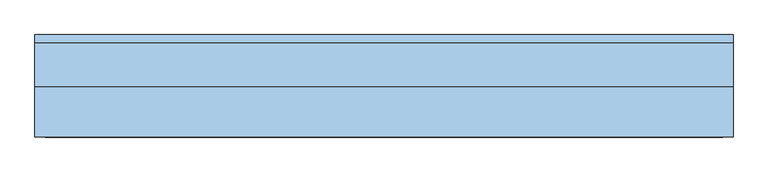
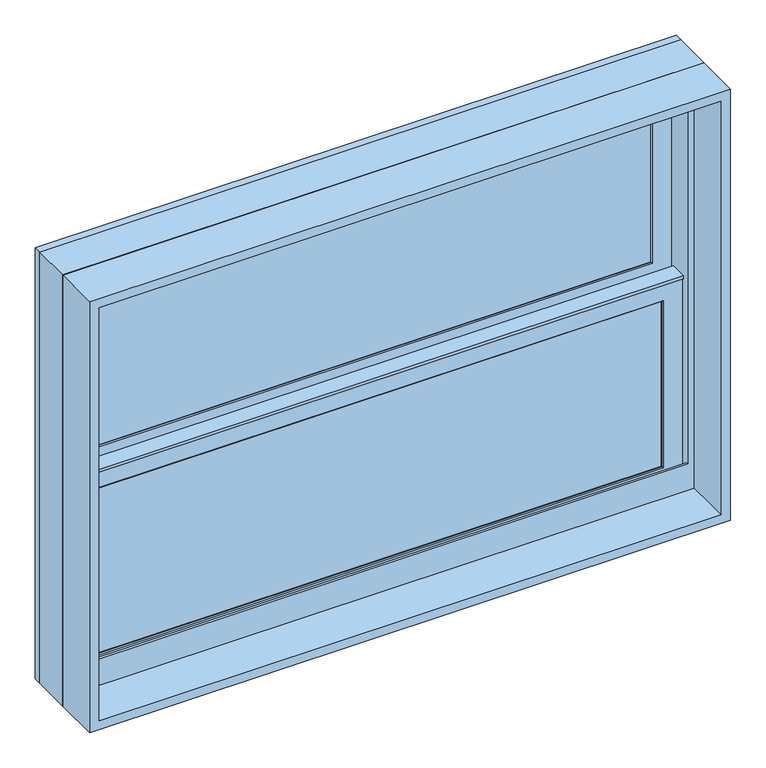
"""IFC4 building model written with IfcOpenShell, lengths in millimetres: window geometry, Window-Double_Hung-Marvin-Essential : ESDH3626."""

from ifc_helpers import new_model, si_unit, frame, origin, place, context, project, spatial, polyline, outline, extrude, faceted_brep, source, transform, mapped, element, save


def window_779252a0(model_context):
    return source(origin(), model_context, "Body", "SolidModel", [
        extrude(outline(polyline([(166.1583333, 20.6375), (166.1583333, 15.875), (147.1083333, 15.875), (147.1083333, 20.6375), (166.1583333, 20.6375)])), frame((0.0, 0.0, 1746.25), z_axis=(0.0, 0.0, 1.0), x_axis=(1.0, 0.0, 0.0)), (0.0, 0.0, 1.0), 298.45),
        extrude(outline(polyline([(-147.1083333, 20.6375), (-147.1083333, 15.875), (-166.1583333, 15.875), (-166.1583333, 20.6375), (-147.1083333, 20.6375)])), frame((0.0, 0.0, 1746.25), z_axis=(0.0, 0.0, 1.0), x_axis=(1.0, 0.0, 0.0)), (0.0, 0.0, 1.0), 298.45),
        extrude(outline(polyline([(469.9, 20.6375), (469.9, 15.875), (-469.9, 15.875), (-469.9, 20.6375), (469.9, 20.6375)])), frame((0.0, 0.0, 1885.95), z_axis=(0.0, 0.0, 1.0), x_axis=(1.0, 0.0, 0.0)), (0.0, 0.0, 1.0), 19.05),
        extrude(outline(polyline([(-166.1583333, 46.83125), (-166.1583333, 51.59375), (-147.1083333, 51.59375), (-147.1083333, 46.83125), (-166.1583333, 46.83125)])), frame((0.0, 0.0, 2082.8), z_axis=(0.0, 0.0, 1.0), x_axis=(1.0, 0.0, 0.0)), (0.0, 0.0, 1.0), 298.45),
        extrude(outline(polyline([(147.1083333, 46.83125), (147.1083333, 51.59375), (166.1583333, 51.59375), (166.1583333, 46.83125), (147.1083333, 46.83125)])), frame((0.0, 0.0, 2082.8), z_axis=(0.0, 0.0, 1.0), x_axis=(1.0, 0.0, 0.0)), (0.0, 0.0, 1.0), 298.45),
        extrude(outline(polyline([(-469.9, 46.83125), (-469.9, 51.59375), (469.9, 51.59375), (469.9, 46.83125), (-469.9, 46.83125)])), frame((0.0, 0.0, 2222.5), z_axis=(0.0, 0.0, 1.0), x_axis=(1.0, 0.0, 0.0)), (0.0, 0.0, 1.0), 19.05),
        extrude(outline(polyline([(166.1583333, 20.6375), (147.1083333, 20.6375), (147.1083333, 25.4), (166.1583333, 25.4), (166.1583333, 20.6375)])), frame((0.0, 0.0, 1746.25), z_axis=(0.0, 0.0, 1.0), x_axis=(1.0, 0.0, 0.0)), (0.0, 0.0, 1.0), 298.45),
        extrude(outline(polyline([(-147.1083333, 20.6375), (-166.1583333, 20.6375), (-166.1583333, 25.4), (-147.1083333, 25.4), (-147.1083333, 20.6375)])), frame((0.0, 0.0, 1746.25), z_axis=(0.0, 0.0, 1.0), x_axis=(1.0, 0.0, 0.0)), (0.0, 0.0, 1.0), 298.45),
        extrude(outline(polyline([(469.9, 20.6375), (-469.9, 20.6375), (-469.9, 25.4), (469.9, 25.4), (469.9, 20.6375)])), frame((0.0, 0.0, 1885.95), z_axis=(0.0, 0.0, 1.0), x_axis=(1.0, 0.0, 0.0)), (0.0, 0.0, 1.0), 19.05),
        extrude(outline(polyline([(-166.1583333, 56.35625), (-147.1083333, 56.35625), (-147.1083333, 51.59375), (-166.1583333, 51.59375), (-166.1583333, 56.35625)])), frame((0.0, 0.0, 2082.8), z_axis=(0.0, 0.0, 1.0), x_axis=(1.0, 0.0, 0.0)), (0.0, 0.0, 1.0), 298.45),
        extrude(outline(polyline([(147.1083333, 56.35625), (166.1583333, 56.35625), (166.1583333, 51.59375), (147.1083333, 51.59375), (147.1083333, 56.35625)])), frame((0.0, 0.0, 2082.8), z_axis=(0.0, 0.0, 1.0), x_axis=(1.0, 0.0, 0.0)), (0.0, 0.0, 1.0), 298.45),
        extrude(outline(polyline([(-469.9, 56.35625), (469.9, 56.35625), (469.9, 51.59375), (-469.9, 51.59375), (-469.9, 56.35625)])), frame((0.0, 0.0, 2222.5), z_axis=(0.0, 0.0, 1.0), x_axis=(1.0, 0.0, 0.0)), (0.0, 0.0, 1.0), 19.05),
        faceted_brep([(-496.8875, 5.6780605, 2074.7351748), (-496.8875, 5.6780605, 2070.1), (496.8875, 5.6780605, 2070.1), (496.8875, 5.6780605, 2074.7351748), (-496.8875, 34.8118605, 2074.7351748), (496.8875, 34.8118605, 2074.7351748), (496.8875, 34.8118605, 2070.1), (-496.8875, 34.8118605, 2070.1), (-496.8875, 30.1625, 2070.1), (-496.8875, 30.1625, 1719.2625), (-496.8875, 8.9241104, 1719.2625), (-496.8875, 8.9241104, 2070.1), (496.8875, 8.9241104, 2070.1), (496.8875, 30.1625, 2070.1), (496.8875, 8.9241104, 1719.2625), (496.8875, 30.1625, 1719.2625), (-481.0034752, 11.90625, 2055.8034752), (-481.0034752, 30.1625, 2055.8034752), (481.0034752, 30.1625, 2055.8034752), (481.0034752, 11.90625, 2055.8034752), (-464.34375, 10.4662439, 2039.14375), (-464.34375, 11.90625, 2039.14375), (464.34375, 11.90625, 2039.14375), (464.34375, 10.4662439, 2039.14375), (465.8858834, 8.9241104, 2040.6858834), (-465.8858834, 8.9241104, 2040.6858834), (481.0034752, 30.1625, 1735.1465248), (481.0034752, 11.90625, 1735.1465248), (464.34375, 11.90625, 1751.80625), (464.34375, 10.4662439, 1751.80625), (465.8858834, 8.9241104, 1750.2641166), (-481.0034752, 30.1625, 1735.1465248), (-481.0034752, 11.90625, 1735.1465248), (-464.34375, 11.90625, 1751.80625), (-464.34375, 10.4662439, 1751.80625), (-465.8858834, 8.9241104, 1750.2641166)], [[[0, 1, 2, 3]], [[4, 5, 6, 7]], [[1, 0, 4, 7, 8, 9, 10, 11]], [[2, 1, 11, 12]], [[7, 6, 13, 8]], [[3, 2, 12, 14, 15, 13, 6, 5]], [[0, 3, 5, 4]], [[16, 17, 18, 19]], [[20, 21, 22, 23]], [[20, 23, 24, 25]], [[19, 18, 26, 27]], [[23, 22, 28, 29]], [[24, 23, 29, 30]], [[27, 26, 31, 32]], [[29, 28, 33, 34]], [[30, 29, 34, 35]], [[15, 14, 10, 9]], [[15, 9, 8, 13], [18, 17, 31, 26]], [[17, 16, 32, 31]], [[16, 19, 27, 32], [22, 21, 33, 28]], [[21, 20, 34, 33]], [[20, 25, 35, 34]], [[10, 14, 12, 11], [25, 24, 30, 35]]]),
        extrude(outline(polyline([(38.5955581, 2055.8125), (33.5778968, 2055.8125), (33.5778968, 2057.4), (39.9405976, 2057.4), (39.9405976, 2055.8125), (61.515625, 2055.8125), (47.6307501, 2052.4975159), (38.5955581, 2052.4975159), (38.5955581, 2055.8125)])), frame((-496.8875, 0.0, 0.0), z_axis=(1.0, 0.0, 0.0), x_axis=(0.0, 1.0, 0.0)), (0.0, 0.0, 1.0), 993.775),
        faceted_brep([(527.05, 0.0, 1689.1), (527.05, 0.0, 2438.4), (-527.05, 0.0, 2438.4), (-527.05, 0.0, 1689.1), (500.85625, 0.0, 1750.21875), (-500.85625, 0.0, 1750.21875), (-500.85625, 0.0, 2412.20625), (500.85625, 0.0, 2412.20625), (500.85625, 3.96875, 1689.1), (-500.85625, 3.96875, 1689.1), (-500.85625, 3.96875, 1750.21875), (500.85625, 3.96875, 1750.21875), (-527.05, 65.6828125, 1689.1), (-500.85625, 65.6828125, 1689.1), (500.85625, 65.6828125, 1689.1), (527.05, 65.6828125, 1689.1), (-527.05, 65.6828125, 2438.4), (527.05, 65.6828125, 2438.4), (500.85625, 65.6828125, 2412.20625), (-500.85625, 65.6828125, 2412.20625)], [[[0, 1, 2, 3], [4, 5, 6, 7]], [[8, 9, 10, 11]], [[5, 4, 11, 10]], [[0, 3, 12, 13, 9, 8, 14, 15]], [[13, 12, 16, 17, 15, 14, 18, 19]], [[13, 19, 6, 5, 10, 9]], [[7, 6, 19, 18]], [[18, 14, 8, 11, 4, 7]], [[1, 0, 15, 17]], [[2, 1, 17, 16]], [[3, 2, 16, 12]]]),
        faceted_brep([(500.85625, 30.1625, 2063.75), (499.26875, 30.1625, 2063.75), (499.26875, 30.1625, 1713.4544613), (500.85625, 30.1625, 1713.4544613), (-499.26875, 30.1625, 2063.75), (-500.85625, 30.1625, 2063.75), (-500.85625, 30.1625, 1713.4544613), (-499.26875, 30.1625, 1713.4544613), (499.26875, 63.5, 2063.75), (500.85625, 63.5, 2063.75), (500.85625, 63.5, 1706.9743077), (499.26875, 63.5, 1706.9743077), (-500.85625, 63.5, 2063.75), (-499.26875, 63.5, 2063.75), (-499.26875, 63.5, 1706.9743077), (-500.85625, 63.5, 1706.9743077), (512.1108932, 3.96875, 1718.5460105), (512.1108932, 3.96875, 1689.1), (512.1108932, 65.6828125, 1689.1), (512.1108932, 65.6828125, 1706.550012), (-512.1108932, 3.96875, 1689.1), (-512.1108932, 3.96875, 1718.5460105), (-512.1108932, 65.6828125, 1706.550012), (-512.1108932, 65.6828125, 1689.1), (512.1108932, 78.58125, 1704.0428097), (-512.1108932, 78.58125, 1704.0428097), (-510.0971252, 68.2348864, 1706.0539391), (-492.13135, 68.2348864, 1706.0539391), (-492.13135, 65.6828125, 1706.550012), (492.13135, 65.6828125, 1706.550012), (492.13135, 68.2348864, 1706.0539391), (510.0971252, 68.2348864, 1706.0539391), (-527.05, 65.6828125, 1689.1), (-527.05, 78.5948249, 1689.1), (527.05, 78.5948249, 1689.1), (527.05, 65.6828125, 1689.1), (-527.05, 78.58125, 2438.4), (527.05, 78.58125, 2438.4), (512.1108932, 78.58125, 2423.4608932), (-512.1108932, 78.58125, 2423.4608932), (-527.05, 65.6828125, 2438.4), (-510.0971252, 68.2348864, 2421.4471252), (510.0971252, 68.2348864, 2421.4471252), (492.13135, 68.2348864, 2403.48135), (-492.13135, 68.2348864, 2403.48135), (-492.13135, 65.6828125, 2403.48135), (492.13135, 65.6828125, 2403.48135), (527.05, 65.6828125, 2438.4)], [[[0, 1, 2, 3]], [[4, 5, 6, 7]], [[8, 9, 10, 11]], [[12, 13, 14, 15]], [[1, 8, 11, 2]], [[9, 0, 3, 10]], [[1, 0, 9, 8]], [[5, 4, 13, 12]], [[5, 12, 15, 6]], [[13, 4, 7, 14]], [[16, 17, 18, 19]], [[20, 21, 22, 23]], [[24, 25, 26, 27, 28, 22, 21, 16, 19, 29, 30, 31], [3, 2, 11, 10], [7, 6, 15, 14]], [[17, 16, 21, 20]], [[17, 20, 23, 32, 33, 34, 35, 18]], [[34, 33, 36, 37], [25, 24, 38, 39]], [[33, 32, 40, 36]], [[39, 41, 26, 25]], [[41, 42, 31, 30, 43, 44, 27, 26]], [[44, 45, 28, 27]], [[40, 32, 23, 22, 28, 45, 46, 29, 19, 18, 35, 47]], [[36, 40, 47, 37]], [[39, 38, 42, 41]], [[44, 43, 46, 45]], [[34, 37, 47, 35]], [[42, 38, 24, 31]], [[46, 43, 30, 29]]]),
        extrude(outline(polyline([(477.04375, 11.90625), (-477.04375, 11.90625), (-477.04375, 15.08125), (477.04375, 15.08125), (477.04375, 11.90625)])), frame((0.0, 0.0, 1739.10625), z_axis=(0.0, 0.0, 1.0), x_axis=(1.0, 0.0, 0.0)), (0.0, 0.0, 1.0), 312.7375),
        extrude(outline(polyline([(477.04375, 42.8625), (-477.04375, 42.8625), (-477.04375, 46.0375), (477.04375, 46.0375), (477.04375, 42.8625)])), frame((0.0, 0.0, 2075.65625), z_axis=(0.0, 0.0, 1.0), x_axis=(1.0, 0.0, 0.0)), (0.0, 0.0, 1.0), 312.7375),
        faceted_brep([(-464.34375, 31.194477, 2039.14375), (-465.8858834, 32.7366104, 2040.6858834), (465.8858834, 32.7366104, 2040.6858834), (464.34375, 31.194477, 2039.14375), (-464.34375, 30.1625, 2039.14375), (464.34375, 30.1625, 2039.14375), (-496.8875, 32.7366104, 2071.6875), (-496.8875, 30.1625, 2071.6875), (496.8875, 30.1625, 2071.6875), (496.8875, 32.7366104, 2071.6875), (465.8858834, 32.7366104, 1750.2641166), (464.34375, 31.194477, 1751.80625), (464.34375, 30.1625, 1751.80625), (496.8875, 30.1625, 1719.2625), (496.8875, 32.7366104, 1719.2625), (-465.8858834, 32.7366104, 1750.2641166), (-464.34375, 31.194477, 1751.80625), (-464.34375, 30.1625, 1751.80625), (-496.8875, 30.1625, 1719.2625), (-496.8875, 32.7366104, 1719.2625)], [[[0, 1, 2, 3]], [[4, 0, 3, 5]], [[6, 7, 8, 9]], [[3, 2, 10, 11]], [[5, 3, 11, 12]], [[9, 8, 13, 14]], [[11, 10, 15, 16]], [[12, 11, 16, 17]], [[14, 13, 18, 19]], [[9, 14, 19, 6], [1, 15, 10, 2]], [[16, 15, 1, 0]], [[17, 16, 0, 4]], [[7, 18, 13, 8], [5, 12, 17, 4]], [[19, 18, 7, 6]]]),
        faceted_brep([(-481.0034752, 42.8625, 2392.3534752), (-481.0034752, 61.11875, 2392.3534752), (481.0034752, 61.11875, 2392.3534752), (481.0034752, 42.8625, 2392.3534752), (-464.34375, 41.4224939, 2375.69375), (-464.34375, 42.8625, 2375.69375), (464.34375, 42.8625, 2375.69375), (464.34375, 41.4224939, 2375.69375), (-465.8858834, 39.8803604, 2377.2358834), (465.8858834, 39.8803604, 2377.2358834), (-496.8875, 61.11875, 2408.2375), (-496.8875, 39.8803604, 2408.2375), (496.8875, 39.8803604, 2408.2375), (496.8875, 61.11875, 2408.2375), (481.0034752, 61.11875, 2071.6965248), (481.0034752, 42.8625, 2071.6965248), (464.34375, 42.8625, 2088.35625), (464.34375, 41.4224939, 2088.35625), (465.8858834, 39.8803604, 2086.8141166), (496.8875, 39.8803604, 2055.8125), (496.8875, 61.11875, 2055.8125), (-481.0034752, 61.11875, 2071.6965248), (-481.0034752, 42.8625, 2071.6965248), (-464.34375, 42.8625, 2088.35625), (-464.34375, 41.4224939, 2088.35625), (-465.8858834, 39.8803604, 2086.8141166), (-496.8875, 39.8803604, 2055.8125), (-496.8875, 61.11875, 2055.8125)], [[[0, 1, 2, 3]], [[4, 5, 6, 7]], [[8, 4, 7, 9]], [[10, 11, 12, 13]], [[3, 2, 14, 15]], [[7, 6, 16, 17]], [[9, 7, 17, 18]], [[13, 12, 19, 20]], [[15, 14, 21, 22]], [[17, 16, 23, 24]], [[18, 17, 24, 25]], [[20, 19, 26, 27]], [[13, 20, 27, 10], [1, 21, 14, 2]], [[22, 21, 1, 0]], [[3, 15, 22, 0], [5, 23, 16, 6]], [[24, 23, 5, 4]], [[25, 24, 4, 8]], [[11, 26, 19, 12], [9, 18, 25, 8]], [[27, 26, 11, 10]]]),
        faceted_brep([(-496.8875, 61.11875, 2055.8125), (-496.8875, 63.6928604, 2055.8125), (496.8875, 63.6928604, 2055.8125), (496.8875, 61.11875, 2055.8125), (-464.34375, 62.150727, 2088.35625), (-464.34375, 61.11875, 2088.35625), (464.34375, 61.11875, 2088.35625), (464.34375, 62.150727, 2088.35625), (-465.8858834, 63.6928604, 2086.8141166), (465.8858834, 63.6928604, 2086.8141166), (496.8875, 63.6928604, 2408.2375), (496.8875, 61.11875, 2408.2375), (464.34375, 61.11875, 2375.69375), (464.34375, 62.150727, 2375.69375), (465.8858834, 63.6928604, 2377.2358834), (-496.8875, 63.6928604, 2408.2375), (-496.8875, 61.11875, 2408.2375), (-464.34375, 61.11875, 2375.69375), (-464.34375, 62.150727, 2375.69375), (-465.8858834, 63.6928604, 2377.2358834)], [[[0, 1, 2, 3]], [[4, 5, 6, 7]], [[8, 4, 7, 9]], [[3, 2, 10, 11]], [[7, 6, 12, 13]], [[9, 7, 13, 14]], [[11, 10, 15, 16]], [[13, 12, 17, 18]], [[14, 13, 18, 19]], [[16, 15, 1, 0]], [[3, 11, 16, 0], [5, 17, 12, 6]], [[18, 17, 5, 4]], [[19, 18, 4, 8]], [[1, 15, 10, 2], [9, 14, 19, 8]]]),
        extrude(outline(polyline([(477.04375, 26.19375), (-477.04375, 26.19375), (-477.04375, 30.1625), (477.04375, 30.1625), (477.04375, 26.19375)])), frame((0.0, 0.0, 1739.10625), z_axis=(0.0, 0.0, 1.0), x_axis=(1.0, 0.0, 0.0)), (0.0, 0.0, 1.0), 312.7375),
        extrude(outline(polyline([(477.04375, 57.15), (-477.04375, 57.15), (-477.04375, 61.11875), (477.04375, 61.11875), (477.04375, 57.15)])), frame((0.0, 0.0, 2075.65625), z_axis=(0.0, 0.0, 1.0), x_axis=(1.0, 0.0, 0.0)), (0.0, 0.0, 1.0), 312.7375),
        extrude(outline(polyline([(2438.4, 527.05), (2438.4, -527.05), (1689.1, -527.05), (1689.1, 527.05), (2438.4, 527.05)]), holes=[polyline([(2422.525, 511.175), (1704.975, 511.175), (1704.975, -511.175), (2422.525, -511.175), (2422.525, 511.175)])]), frame((0.0, -76.2, 0.0), z_axis=(0.0, 1.0, 0.0), x_axis=(0.0, 0.0, 1.0)), (0.0, 0.0, 1.0), 75.40625),
    ])


if __name__ == "__main__":
    model = new_model("IFC4")
    model_context = context("Model", 3, world=origin())
    ifc_project = project(units=[si_unit("LENGTHUNIT", "METRE", prefix="MILLI")], contexts=[model_context])
    site = spatial("IfcSite", under=ifc_project)
    building = spatial("IfcBuilding", under=site)
    placement = place(None, origin())
    window_shape = window_779252a0(model_context)
    element("IfcWindow", 1, ObjectType="Window-Double_Hung-Marvin-Essential : ESDH3626", at=placement, inside=building, context=model_context, shape_type="MappedRepresentation", body=[
        mapped(window_shape, transform((0.0, 0.0, 0.0), x_axis=(1.0, 0.0, 0.0), y_axis=(0.0, 1.0, 0.0), z_axis=(0.0, 0.0, 1.0))),
    ])
    save(model, "model.ifc")

# Revit data of these elements
# Type "Window-Double_Hung-Marvin-Essential : ESDH3626"
#   Type Mark = "31"
#   Window Type = "Essential Double Hung"
#   Product data url = "https://bimobject.com/marvin-windows-and-doors/product/marvin-dhwau"
#   Product Guid = "c4a96547-874c-4385-91dc-a058adc19d98"
#   Frame = "All Ultrex"
#   Egress Window = "No"
#   URL = "www.marvin.com"
#   Model = "ESDH3626"
#   Manufacturer = "Marvin Windows and Doors"
#   Label Egress = ""
#   Glass Type = "IG Low E II with Argon"
#   Design Pressure = "DP50"
#   Description = "4230 DBHG"
#   Analytic Construction = "<None>"
#   Prairie Corner Width = 0' - 4"
#   Prairie Corner Height = 0' - 4"
#   Egress Width = 3' - 2 9/16"
#   Egress Height = 0' - 10 27/128"
#   Rough Width = 3' - 6"
#   Rough Height = 2' - 6"
#   Nominal Width = 3' - 6"
#   Nominal Height = 2' - 6"
#   Inset to Installation Flange [instance default] = 0' - 1"
#   Height = 2' - 5 1/2"
#   Egress Area = 2.73444 SF
#   Default Head Height = 8' - 0"
#   Width = 3' - 5 1/2"
#   Daylight Area = 5.74463 SF
#   DLO Width = 3' - 0 9/16"
#   DLO Height = 0' - 11 5/16"
#   Muntins Top Sash = yes
#   Lites Wide Top Sash = 3
#   Lites Wide Bottom Sash = 3
#   Lites High Top Sash = 2
#   Lites High Bottom Sash = 2
#   Lite Cut Prairie 9 = no
#   Lite Cut HV Grid = yes
#   Muntins Bottom Sash = yes
#   Label Visibility = no
#   Jamb Extension Visibility = yes
#   Edition number = 1
#   Interior Material = Ultrex-Marvin-Stonewhite
#   Glazing Material = Glass-Marvin-IG Low E II with Argon
#   Cladding Material = Ultrex-Marvin-Pebblegray
#   Wall Closure = (empty or 0)
#   Assembly Code = ""
# Element 1 (IfcWindow, "Window-Double_Hung-Marvin-Essential : ESDH3626")
#   Materials on its faces: "Ultrex-Marvin-Pebblegray", "Ultrex-Marvin-Stonewhite", "Glass-Marvin-IG Low E II with Argon"
# Materials
#   "Ultrex-Marvin-Stonewhite": class "Paint", colour RGB 250 251 245, transparency 0
#   "Glass-Marvin-IG Low E II with Argon": class "Glass", colour RGB 0 128 192, transparency 0.85
#   "Ultrex-Marvin-Pebblegray": class "Paint", colour RGB 189 185 173, transparency 0
